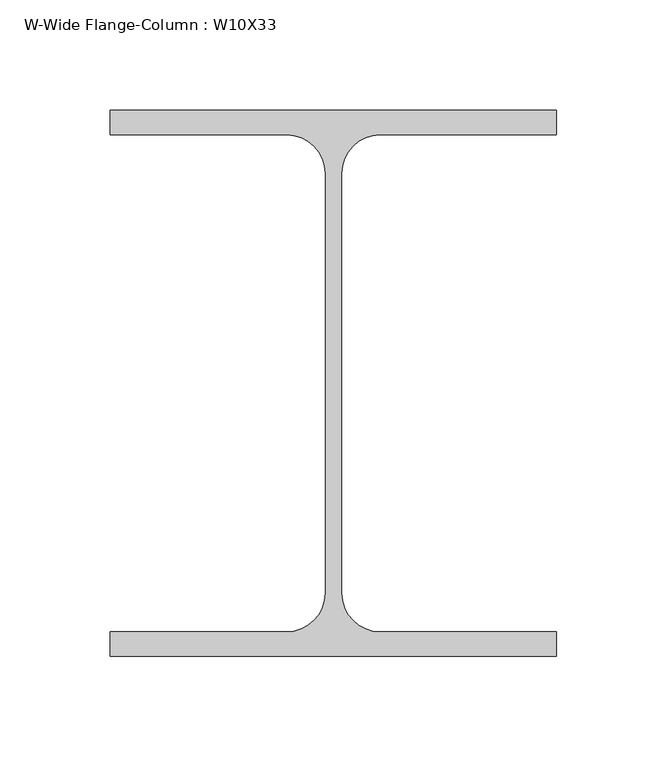
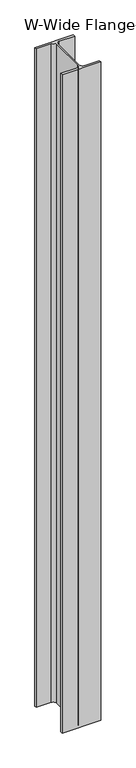
"""IFC4 building model written with IfcOpenShell, lengths in millimetres: column geometry, W-Wide Flange-Column : W10X33."""

from ifc_helpers import new_model, si_unit, point, frame, frame_2d, origin, place, context, project, spatial, polyline, circle_curve, trimmed, segment, composite_curve, outline, extrude, source, transform, mapped, element, save


def w_wide_flange_column_w10x33_bc32e965(model_context):
    return source(origin(), model_context, "Body", "SweptSolid", [
        extrude(outline(composite_curve([segment(polyline([(101.092, 123.571), (101.092, 112.522), (21.209, 112.522)]), True, "CONTINUOUS"), segment(trimmed(circle_curve(frame_2d((21.209, 94.996)), 17.526), [point((21.209, 112.522))], [point((3.683, 94.996))], True, "CARTESIAN"), True, "CONTINUOUS"), segment(polyline([(3.683, 94.996), (3.683, -94.996)]), True, "CONTINUOUS"), segment(trimmed(circle_curve(frame_2d((21.209, -94.996)), 17.526), [point((3.683, -94.996))], [point((21.209, -112.522))], True, "CARTESIAN"), True, "CONTINUOUS"), segment(polyline([(21.209, -112.522), (101.092, -112.522), (101.092, -123.571), (-101.092, -123.571), (-101.092, -112.522), (-21.209, -112.522)]), True, "CONTINUOUS"), segment(trimmed(circle_curve(frame_2d((-21.209, -94.996)), 17.526), [point((-21.209, -112.522))], [point((-3.683, -94.996))], True, "CARTESIAN"), True, "CONTINUOUS"), segment(polyline([(-3.683, -94.996), (-3.683, 94.996)]), True, "CONTINUOUS"), segment(trimmed(circle_curve(frame_2d((-21.209, 94.996)), 17.526), [point((-3.683, 94.996))], [point((-21.209, 112.522))], True, "CARTESIAN"), True, "CONTINUOUS"), segment(polyline([(-21.209, 112.522), (-101.092, 112.522), (-101.092, 123.571), (101.092, 123.571)]), True, "CONTINUOUS")], self_intersect=False)), frame((0.0, 0.0, 8756.65), z_axis=(0.0, 0.0, 1.0), x_axis=(1.0, 0.0, 0.0)), (0.0, 0.0, 1.0), 3651.25),
    ])


if __name__ == "__main__":
    model = new_model("IFC4")
    model_context = context("Model", 3, world=origin())
    ifc_project = project(units=[si_unit("LENGTHUNIT", "METRE", prefix="MILLI")], contexts=[model_context])
    site = spatial("IfcSite", under=ifc_project)
    building = spatial("IfcBuilding", under=site)
    placement = place(None, origin())
    w_wide_flange_column_w10x33_shape = w_wide_flange_column_w10x33_bc32e965(model_context)
    element("IfcColumn", 1, ObjectType="W-Wide Flange-Column : W10X33", at=placement, inside=building, context=model_context, shape_type="MappedRepresentation", body=[
        mapped(w_wide_flange_column_w10x33_shape, transform((0.0, 0.0, 0.0), x_axis=(1.0, 0.0, 0.0), y_axis=(0.0, 1.0, 0.0), z_axis=(0.0, 0.0, 1.0))),
    ])
    save(model, "model.ifc")

# Revit data of these elements
# Type "W-Wide Flange-Column : W10X33"
#   Assembly Code = "B10"
#   W = 33
#   bf = 0' - 7.96"
#   d = 0' - 9.73"
#   k = 0' - 1 1/8"
#   kr = 0' - 0.69"
#   tf = 0' - 0.435"
#   tw = 0' - 0.29"
#   A = 0.0674306 SF
#   Structural Material [instance default] = Steel ASTM A992
# Element 1 (IfcColumn, "W-Wide Flange-Column : W10X33")
#   Materials on its faces: "Steel ASTM A992"
# Materials
#   "Steel ASTM A992": class "Metal", colour RGB 199 199 199, transparency 0, Description = "Structural steel 50ksi", Cost = 0
